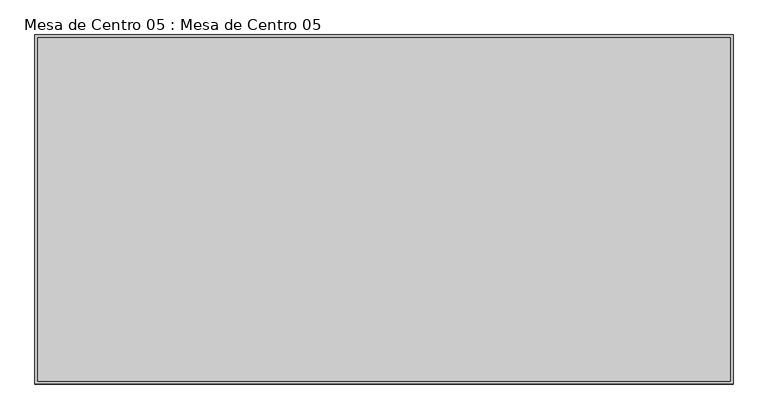
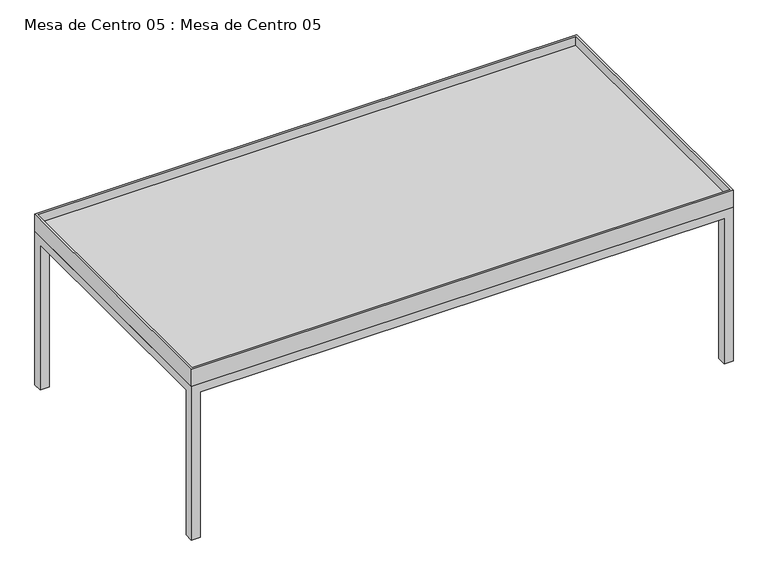
"""IFC4 building model written with IfcOpenShell, lengths in millimetres: proxy geometry, Mesa de Centro 05 : Mesa de Centro 05."""

from ifc_helpers import new_model, si_unit, origin, place, context, project, spatial, faceted_brep, source, transform, mapped, element, save


def mesa_de_centro_05_mesa_de_centro_05_ed090e41(model_context):
    return source(origin(), model_context, "Body", "Brep", [
        faceted_brep([(600.0, 300.0, 360.0), (600.0, 300.0, 400.0), (600.0, -300.0, 400.0), (600.0, -300.0, 360.0), (595.0, 295.0, 400.0), (595.0, 295.0, 380.0), (595.0, -295.0, 380.0), (595.0, -295.0, 400.0), (-600.0, -300.0, 400.0), (-600.0, -300.0, 360.0), (-595.0, -295.0, 380.0), (-595.0, -295.0, 400.0), (-600.0, 300.0, 400.0), (-600.0, 300.0, 360.0), (-595.0, 295.0, 380.0), (-595.0, 295.0, 400.0)], [[[0, 1, 2, 3]], [[4, 5, 6, 7]], [[3, 2, 8, 9]], [[7, 6, 10, 11]], [[9, 8, 12, 13]], [[11, 10, 14, 15]], [[1, 0, 13, 12]], [[0, 3, 9, 13]], [[6, 5, 14, 10]], [[5, 4, 15, 14]], [[2, 1, 12, 8], [4, 7, 11, 15]]]),
        faceted_brep([(600.0, 300.0, 360.0), (-600.0, 300.0, 360.0), (-600.0, -300.0, 360.0), (600.0, -300.0, 360.0), (580.0, 280.0, 360.0), (580.0, -280.0, 360.0), (-580.0, -280.0, 360.0), (-580.0, 280.0, 360.0), (580.0, 280.0, 340.0), (-580.0, 280.0, 340.0), (-580.0, 300.0, 340.0), (580.0, 300.0, 340.0), (-580.0, -280.0, 340.0), (-600.0, -280.0, 340.0), (-600.0, 280.0, 340.0), (580.0, -280.0, 340.0), (580.0, -300.0, 340.0), (-580.0, -300.0, 340.0), (600.0, 280.0, 340.0), (600.0, -280.0, 340.0), (600.0, 300.0, 0.0), (580.0, 300.0, 0.0), (-580.0, 300.0, 0.0), (-600.0, 300.0, 0.0), (-600.0, 280.0, 0.0), (-600.0, -280.0, 0.0), (-600.0, -300.0, 0.0), (-580.0, -300.0, 0.0), (580.0, -300.0, 0.0), (600.0, -300.0, 0.0), (600.0, -280.0, 0.0), (600.0, 280.0, 0.0), (580.0, 280.0, 0.0), (-580.0, -280.0, 0.0), (-580.0, 280.0, 0.0), (580.0, -280.0, 0.0)], [[[0, 1, 2, 3], [4, 5, 6, 7]], [[8, 9, 10, 11]], [[9, 12, 13, 14]], [[12, 15, 16, 17]], [[15, 8, 18, 19]], [[1, 0, 20, 21, 11, 10, 22, 23]], [[2, 1, 23, 24, 14, 13, 25, 26]], [[3, 2, 26, 27, 17, 16, 28, 29]], [[20, 0, 3, 29, 30, 19, 18, 31]], [[5, 4, 8, 15]], [[6, 5, 15, 12]], [[7, 6, 12, 9]], [[4, 7, 9, 8]], [[21, 20, 31, 32]], [[27, 26, 25, 33]], [[22, 34, 24, 23]], [[28, 35, 30, 29]], [[24, 34, 9, 14]], [[34, 22, 10, 9]], [[21, 32, 8, 11]], [[32, 31, 18, 8]], [[27, 33, 12, 17]], [[33, 25, 13, 12]], [[30, 35, 15, 19]], [[35, 28, 16, 15]]]),
    ])


if __name__ == "__main__":
    model = new_model("IFC4")
    model_context = context("Model", 3, world=origin())
    ifc_project = project(units=[si_unit("LENGTHUNIT", "METRE", prefix="MILLI")], contexts=[model_context])
    site = spatial("IfcSite", under=ifc_project)
    building = spatial("IfcBuilding", under=site)
    placement = place(None, origin())
    mesa_de_centro_05_mesa_de_centro_05_shape = mesa_de_centro_05_mesa_de_centro_05_ed090e41(model_context)
    element("IfcBuildingElementProxy", 1, Name="Mesa de Centro 05 : Mesa de Centro 05", ObjectType="Mesa de Centro 05 : Mesa de Centro 05", at=placement, inside=building, context=model_context, shape_type="MappedRepresentation", body=[
        mapped(mesa_de_centro_05_mesa_de_centro_05_shape, transform((0.0, 0.0, 0.0), x_axis=(1.0, 0.0, 0.0), y_axis=(0.0, 1.0, 0.0), z_axis=(0.0, 0.0, 1.0))),
    ])
    save(model, "model.ifc")

# Revit data of these elements
# Type "Mesa de Centro 05 : Mesa de Centro 05"
#   URL = "www.vitrinerevit.com"
#   Description = "Baixe famílias gratuitas no site!"
#   Largura = 600 mm
#   Comprimento = 1200 mm
#   Altura = 400 mm
#   Material Superior = Laca Branca
#   Material Pés = Wood (Oak)
# Element 1 (IfcBuildingElementProxy, "Mesa de Centro 05 : Mesa de Centro 05")
#   Materials on its faces: "Wood (Oak)", "Laca Branca"
# Materials
#   "Laca Branca": class "Generic", colour RGB 255 255 255, transparency 0, Cost = 0
#   "Wood (Oak)": class "Wood", colour RGB 132 88 61, transparency 0, Description = "physical material", Cost = 0
